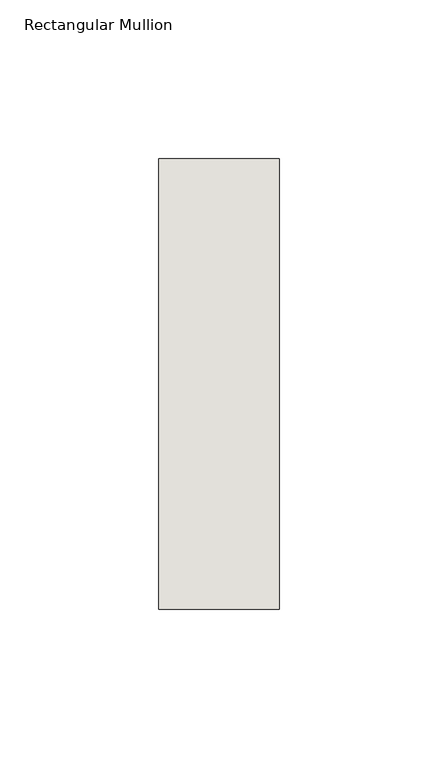
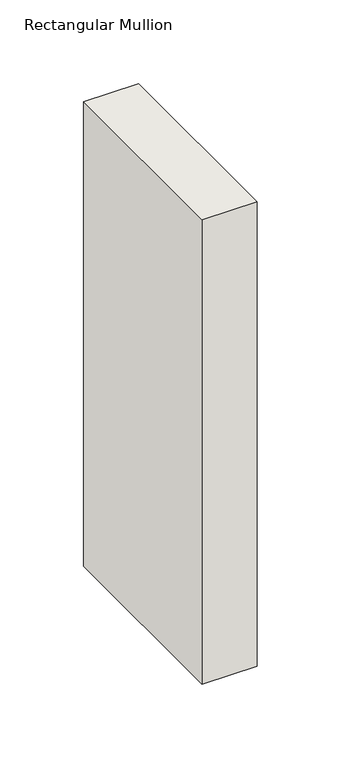
"""IFC4 building model written with IfcOpenShell, lengths in millimetres: wall geometry, Rectangular Mullion : NLRS_21_CWM_hsb-regel 38x142_gen_rsf."""

import ifcopenshell
import ifcopenshell.guid

model = None  # the IFC model being written
_history = None  # IfcOwnerHistory: only IFC2X3 demands one
_inside = {}  # id of a spatial element -> (the spatial element, [elements in it])
_under = {}  # id of a project, library or spatial element -> (it, [spatial elements below it])
_declared = {}  # id of a project -> (the project, [libraries it declares])
_typed = {}  # id of a type object -> (the type object, [elements of that type])
_made_of = {}  # id of a material, layer set ... -> (it, [elements and type objects made of it])


def new_model(schema):
    """Start an empty IFC model of exactly this schema.

    Asked for "IFC4X3", IfcOpenShell would pick the latest addendum, in which some entities
    have other attributes; the version numbers below select the first issue.
    IFC2X3 requires an IfcOwnerHistory on every rooted entity: one is made here for all.
    """
    global model, _history
    if schema == "IFC4X3":
        model = ifcopenshell.file(schema_version=(4, 3, 0, 0))
    else:
        model = ifcopenshell.file(schema=schema)
    _inside.clear()
    _under.clear()
    _declared.clear()
    _typed.clear()
    _made_of.clear()
    _history = None
    if model.schema == "IFC2X3":
        org = make("IfcOrganization", Name="unknown")
        user = make(
            "IfcPersonAndOrganization",
            ThePerson=make("IfcPerson", FamilyName="unknown"),
            TheOrganization=org,
        )
        app = make(
            "IfcApplication",
            ApplicationDeveloper=org,
            Version="unknown",
            ApplicationFullName="unknown",
            ApplicationIdentifier="unknown",
        )
        _history = make(
            "IfcOwnerHistory",
            OwningUser=user,
            OwningApplication=app,
            ChangeAction="ADDED",
            CreationDate=0,
        )
    return model


def make(cls, **values):
    """One entity of the class cls with the attributes given. An attribute that is None is left unset."""
    return model.create_entity(
        cls, **{name: value for name, value in values.items() if value is not None}
    )


def rooted(cls, **values):
    """An entity with a GlobalId (a new one), such as an element, a storey or a relation."""
    return make(cls, GlobalId=ifcopenshell.guid.new(), OwnerHistory=_history, **values)


def si_unit(unit_type, name, prefix=None):
    """IfcSIUnit, for example si_unit("LENGTHUNIT", "METRE", prefix="MILLI")."""
    return make("IfcSIUnit", UnitType=unit_type, Prefix=prefix, Name=name)


def assignment(units):
    """IfcUnitAssignment: the units of a project."""
    return None if units is None else make("IfcUnitAssignment", Units=units)


def point(xyz):
    """IfcCartesianPoint."""
    return None if xyz is None else make("IfcCartesianPoint", Coordinates=xyz)


def direction(xyz):
    """IfcDirection."""
    return None if xyz is None else make("IfcDirection", DirectionRatios=xyz)


def frame(location, z_axis=None, x_axis=None):
    """IfcAxis2Placement3D, a coordinate frame: its origin and axes. An axis left out is left unset."""
    return make(
        "IfcAxis2Placement3D",
        Location=point(location),
        Axis=direction(z_axis),
        RefDirection=direction(x_axis),
    )


def origin():
    """The frame at (0, 0, 0) with its axes left unset."""
    return frame((0.0, 0.0, 0.0))


def place(relative_to, where):
    """IfcLocalPlacement: puts the frame where relative to a parent placement (None: the world)."""
    return make(
        "IfcLocalPlacement", PlacementRelTo=relative_to, RelativePlacement=where
    )


def context(
    kind, dimensions, precision=None, world=None, true_north=None, identifier=None
):
    """IfcGeometricRepresentationContext, for example the 3D "Model" context."""
    return make(
        "IfcGeometricRepresentationContext",
        ContextIdentifier=identifier,
        ContextType=kind,
        CoordinateSpaceDimension=dimensions,
        Precision=precision,
        WorldCoordinateSystem=world,
        TrueNorth=true_north,
    )


def project(units=None, contexts=None):
    """IfcProject with its units and contexts."""
    return rooted(
        "IfcProject",
        Name="project",
        RepresentationContexts=contexts,
        UnitsInContext=assignment(units),
    )


def spatial(cls, under=None, at=None, **own):
    """A site, building, storey or space (cls), placed at a placement, below another one or the project."""
    s = rooted(cls, ObjectPlacement=at, **own)
    if under is not None:
        _under.setdefault(under.id(), (under, []))[1].append(s)
    return s


def polyline(points):
    """IfcPolyline through the points."""
    return make("IfcPolyline", Points=[point(p) for p in points])


def outline(outer, holes=None, kind="AREA"):
    """IfcArbitraryClosedProfileDef: a profile drawn as a closed curve; with holes, ...WithVoids."""
    if holes is None:
        return make("IfcArbitraryClosedProfileDef", ProfileType=kind, OuterCurve=outer)
    return make(
        "IfcArbitraryProfileDefWithVoids",
        ProfileType=kind,
        OuterCurve=outer,
        InnerCurves=holes,
    )


def extrude(swept, where, along, depth):
    """IfcExtrudedAreaSolid: the profile swept, set in the frame where, extruded along a direction by depth."""
    return make(
        "IfcExtrudedAreaSolid",
        SweptArea=swept,
        Position=where,
        ExtrudedDirection=direction(along),
        Depth=depth,
    )


def shape(context_of_items, identifier, shape_type, items):
    """IfcShapeRepresentation: the items that make up one representation, for example the "Body"."""
    return make(
        "IfcShapeRepresentation",
        ContextOfItems=context_of_items,
        RepresentationIdentifier=identifier,
        RepresentationType=shape_type,
        Items=items,
    )


def source(mapping_origin, context_of_items, identifier, shape_type, items):
    """IfcRepresentationMap: a shape defined once, which mapped items show again and again."""
    return make(
        "IfcRepresentationMap",
        MappingOrigin=mapping_origin,
        MappedRepresentation=shape(context_of_items, identifier, shape_type, items),
    )


def transform(
    local_origin,
    x_axis=None,
    y_axis=None,
    z_axis=None,
    scale=None,
    scale2=None,
    scale3=None,
    uniform=True,
):
    """IfcCartesianTransformationOperator3D, or its non-uniform kind. x_axis, y_axis, z_axis: its Axis1, 2, 3."""
    if uniform:
        return make(
            "IfcCartesianTransformationOperator3D",
            Axis1=direction(x_axis),
            Axis2=direction(y_axis),
            LocalOrigin=point(local_origin),
            Scale=scale,
            Axis3=direction(z_axis),
        )
    return make(
        "IfcCartesianTransformationOperator3DnonUniform",
        Axis1=direction(x_axis),
        Axis2=direction(y_axis),
        LocalOrigin=point(local_origin),
        Scale=scale,
        Axis3=direction(z_axis),
        Scale2=scale2,
        Scale3=scale3,
    )


def mapped(mapping_source, mapping_target):
    """IfcMappedItem: shows the shape of a source again, moved by a transform."""
    return make(
        "IfcMappedItem", MappingSource=mapping_source, MappingTarget=mapping_target
    )


def made_of(thing, what):
    """Note that an element or type object is made of a material, layer set ...; save() writes the relation."""
    if what is not None:
        _made_of.setdefault(what.id(), (what, []))[1].append(thing)
    return thing


def element(
    cls,
    number,
    at=None,
    inside=None,
    cuts=None,
    type_object=None,
    material=None,
    context=None,
    identifier="Body",
    shape_type=None,
    held_by="IfcProductDefinitionShape",
    body=None,
    shapes=None,
    **own,
):
    """One element of the class cls, such as IfcWall. Its Tag is "e" and its number.

    at: its placement. inside: the storey or other place that contains it. cuts: it is an
    opening in that element (IfcRelVoidsElement). A single representation is given by context,
    identifier, shape_type and body (its items); several are given by shapes. held_by: the class
    of the entity that holds the representations. save() writes the other relations.
    """
    e = rooted(cls, Tag="e%d" % number, ObjectPlacement=at, **own)
    if body is not None:
        shapes = [shape(context, identifier, shape_type, body)]
    if shapes is not None:
        e.Representation = make(held_by, Representations=shapes)
    if inside is not None:
        _inside.setdefault(inside.id(), (inside, []))[1].append(e)
    if cuts is not None:
        rooted(
            "IfcRelVoidsElement", RelatingBuildingElement=cuts, RelatedOpeningElement=e
        )
    if type_object is not None:
        _typed.setdefault(type_object.id(), (type_object, []))[1].append(e)
    return made_of(e, material)


def aggregate(whole, parts):
    """IfcRelAggregates: a whole, such as a stair, and the parts it consists of."""
    return rooted("IfcRelAggregates", RelatingObject=whole, RelatedObjects=parts)


def save(model, path):
    """Write the relations noted so far, then the file.

    IfcRelAggregates (storeys below a building ...), IfcRelContainedInSpatialStructure (elements
    in a storey), IfcRelDefinesByType, IfcRelAssociatesMaterial and IfcRelDeclares: one each for
    every whole, place, type object, material and project.
    """
    for whole, parts in _under.values():
        aggregate(whole, parts)
    for where, things in _inside.values():
        rooted(
            "IfcRelContainedInSpatialStructure",
            RelatedElements=things,
            RelatingStructure=where,
        )
    for kind, things in _typed.values():
        rooted("IfcRelDefinesByType", RelatedObjects=things, RelatingType=kind)
    for what, things in _made_of.values():
        rooted("IfcRelAssociatesMaterial", RelatedObjects=things, RelatingMaterial=what)
    for by, libraries in _declared.values():
        rooted("IfcRelDeclares", RelatingContext=by, RelatedDefinitions=libraries)
    model.write(path)


def rectangular_mullion_1e8108f6(model_context):
    return source(origin(), model_context, "Body", "SweptSolid", [
        extrude(outline(polyline([(19.0, -71.0), (-19.0, -71.0), (-19.0, 71.0), (19.0, 71.0), (19.0, -71.0)])), frame((0.0, 0.0, -339.0041412), z_axis=(0.0, 0.0, 1.0), x_axis=(1.0, 0.0, 0.0)), (0.0, 0.0, 1.0), 339.0041412),
    ])


if __name__ == "__main__":
    model = new_model("IFC4")
    model_context = context("Model", 3, world=origin())
    ifc_project = project(units=[si_unit("LENGTHUNIT", "METRE", prefix="MILLI")], contexts=[model_context])
    site = spatial("IfcSite", under=ifc_project)
    building = spatial("IfcBuilding", under=site)
    placement = place(None, origin())
    rectangular_mullion_shape = rectangular_mullion_1e8108f6(model_context)
    element("IfcWall", 1, ObjectType="Rectangular Mullion : NLRS_21_CWM_hsb-regel 38x142_gen_rsf", at=placement, inside=building, context=model_context, shape_type="MappedRepresentation", body=[
        mapped(rectangular_mullion_shape, transform((0.0, 0.0, 0.0), x_axis=(1.0, 0.0, 0.0), y_axis=(0.0, 1.0, 0.0), z_axis=(0.0, 0.0, 1.0))),
    ])
    save(model, "model.ifc")

# Revit data of these elements
# Type "Rectangular Mullion : NLRS_21_CWM_hsb-regel 38x142_gen_rsf"
#   Type IfcGUID = "07M7mRoiH1CR8m_RSKIwpF"
#   Assembly Code = "21.10"
#   IfcExportAs = "IfcWall"
#   built-in parameter 1007322 = 0.465879 (stored number, unit not read)
#   built-in parameter 1007321 = 0.062336 (stored number, unit not read)
#   built-in parameter 1007320 = 0.062336 (stored number, unit not read)
# Element 1 (IfcWall, "Rectangular Mullion : NLRS_21_CWM_hsb-regel 38x142_gen_rsf")
#   Materials on its faces: "NLRS_i2_hout naaldhout vuren_gen_rsf"
# Materials
#   "NLRS_i2_hout naaldhout vuren_gen_rsf": class "I - Hout", colour RGB 234 199 147, transparency 0, Keynote = "i2", Manufacturer = "Revit Standards Foundation", URL = "www.revitstandards.org", Description = "hout vuren", Cost = 0
